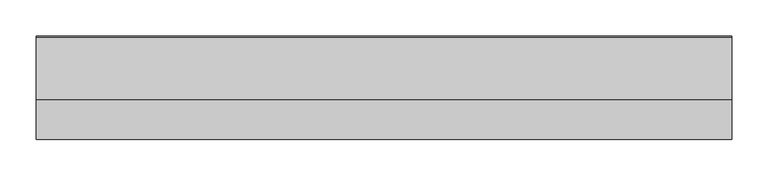
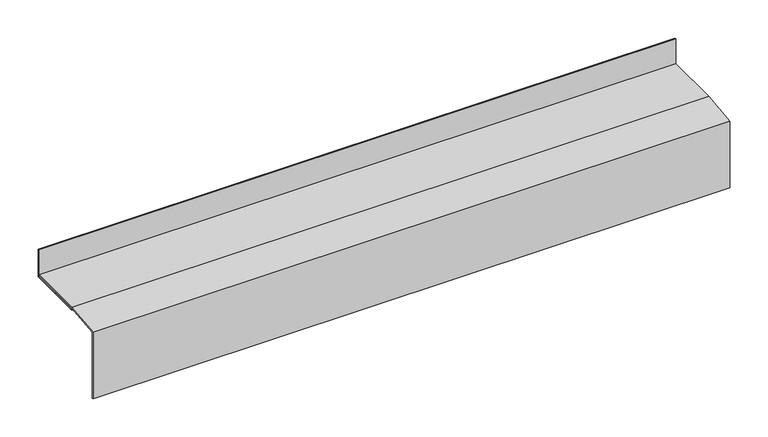
"""IFC4 building model written with IfcOpenShell, lengths in millimetres: proxy geometry, Generic Models 7:Generic Models 1:7:Generic Models 1:7 : Generic Models 7:Generic Models 1:337419:6 : Generic Models 7:Generic Models 1:7:Generic Models 1:7 : Generic Models 7:Generic Models 1:337419:315055."""

from ifc_helpers import new_model, si_unit, frame, origin, place, context, project, spatial, polyline, outline, extrude, source, transform, mapped, element, save


def generic_models_16831a0a(model_context):
    return source(origin(), model_context, "Body", "SweptSolid", [
        extrude(outline(polyline([(-579144.8160706, -81.7582633), (-579144.8160706, 24.2909738), (-579089.3872692, 30.4457208), (-579003.8194128, 30.4457208), (-579003.8194128, 28.8582208), (-579089.2994022, 28.8582208), (-579143.2285706, 22.8699913), (-579143.2285706, -81.7582633), (-579144.8160706, -81.7582633)])), frame((569470.2262575, 0.0, 0.0), z_axis=(1.0, 0.0, 0.0), x_axis=(0.0, 1.0, 0.0)), (0.0, 0.0, 1.0), 961.1225009),
        extrude(outline(polyline([(-579002.9968291, 27.0981204), (-579002.9968291, 69.9933987), (-579001.4093291, 69.9933987), (-579001.4093291, 25.5106204), (-579089.5913841, 25.5106204), (-579089.5913841, 27.0981204), (-579002.9968291, 27.0981204)])), frame((569470.2262575, 0.0, 0.0), z_axis=(1.0, 0.0, 0.0), x_axis=(0.0, 1.0, 0.0)), (0.0, 0.0, 1.0), 961.1225009),
    ])


if __name__ == "__main__":
    model = new_model("IFC4")
    model_context = context("Model", 3, world=origin())
    ifc_project = project(units=[si_unit("LENGTHUNIT", "METRE", prefix="MILLI")], contexts=[model_context])
    site = spatial("IfcSite", under=ifc_project)
    building = spatial("IfcBuilding", under=site)
    placement = place(None, origin())
    generic_models_shape = generic_models_16831a0a(model_context)
    element("IfcBuildingElementProxy", 1, Name="Generic Models 7:Generic Models 1:7:Generic Models 1:7 : Generic Models 7:Generic Models 1:337419:6 : Generic Models 7:Generic Models 1:7:Generic Models 1:7 : Generic Models 7:Generic Models 1:337419:315055", ObjectType="Generic Models 7:Generic Models 1:7:Generic Models 1:7 : Generic Models 7:Generic Models 1:337419:6 : Generic Models 7:Generic Models 1:7:Generic Models 1:7 : Generic Models 7:Generic Models 1:337419:315055", at=placement, inside=building, context=model_context, shape_type="MappedRepresentation", body=[
        mapped(generic_models_shape, transform((0.0, 0.0, 0.0), x_axis=(1.0, 0.0, 0.0), y_axis=(0.0, 1.0, 0.0), z_axis=(0.0, 0.0, 1.0))),
    ])
    save(model, "model.ifc")

# Revit data of these elements
# Type "Generic Models 7:Generic Models 1:7:Generic Models 1:7 : Generic Models 7:Generic Models 1:337419:6 : Generic Models 7:Generic Models 1:7:Generic Models 1:7 : Generic Models 7:Generic Models 1:337419:315055"
#   NameOverride = "Generic Models 7:Generic Models 1:7:Generic Models 1:7 : Generic Models 7:Generic Models 1:337419:315055"
#   ObjectTypeOverride = "Generic Models 1:7 : Generic Models 7:Generic Models 1:337419"
#   Reference = "Generic Models 1"
#   Tag = "315055"
# Element 1 (IfcBuildingElementProxy, "Generic Models 7:Generic Models 1:7:Generic Models 1:7 : Generic Models 7:Generic Models 1:337419:6 : Generic Models 7:Generic Models 1:7:Generic Models 1:7 : Generic Models 7:Generic Models 1:337419:315055")
#   Materials on its faces: "ANODIZED ALUM. FLASHING - MATCH STOREFRONT (ALIGN WITH OTHER WALL ASSEMBLIES)"
# Materials
#   "ANODIZED ALUM. FLASHING - MATCH STOREFRONT (ALIGN WITH OTHER WALL ASSEMBLIES)": class "Unassigned", colour RGB 210 209 208, transparency 0, Cost = 0
